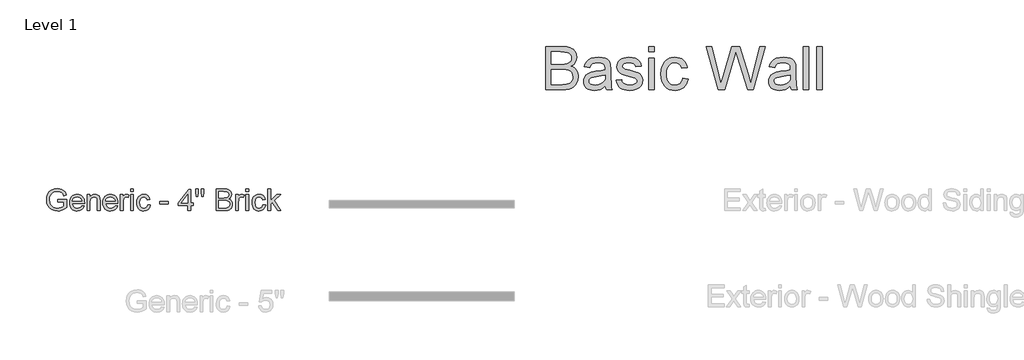
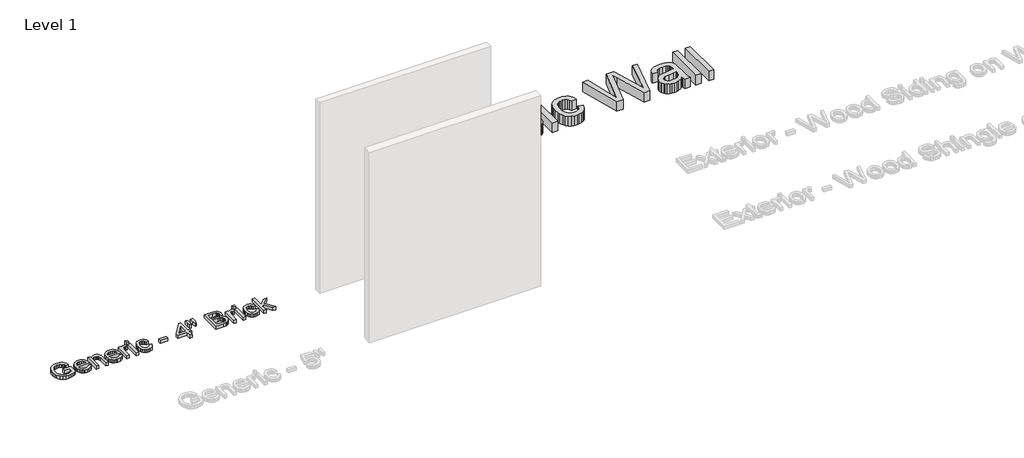
# One storey, part 29 of 42: 2 proxies.
"""IFC4 building model written with IfcOpenShell, lengths in millimetres."""

from ifc_helpers import new_model, si_unit, origin, origin_with_axes, place, context, project, spatial, polyline, outline, extrude, element, save

model = new_model("IFC4")

# Units and contexts
model_context = context("Model", 3, world=origin())
ifc_project = project(units=[si_unit("LENGTHUNIT", "METRE", prefix="MILLI")], contexts=[model_context])

# Site, building, storey
site = spatial("IfcSite", under=ifc_project)
building = spatial("IfcBuilding", under=site)
storey = spatial("IfcBuildingStorey", under=building, Name="Level 1", Elevation=0.0)

# Proxies
placement = place(None, origin())
element("IfcBuildingElementProxy", 1, Name="24\" Arial", ObjectType="24\" Arial", at=placement, inside=storey, context=model_context, shape_type="SweptSolid", body=[
    extrude(outline(polyline([(-9488.2762734, 19004.6336084), (-9488.2762734, 19613.7677966), (-9255.835664, 19613.7677966), (-9191.9070607, 19609.2877752), (-9141.9947897, 19595.8477112), (-9121.7045686, 19585.6840113), (-9103.73801, 19573.1129971), (-9088.0951139, 19558.1346685), (-9074.7758803, 19540.7490255), (-9056.5397768, 19502.6781387), (-9050.4610757, 19462.8226792), (-9055.5731332, 19426.1459899), (-9070.9093059, 19391.6628381), (-9096.5811294, 19361.4924039), (-9132.7001396, 19337.7538676), (-9109.7191173, 19327.9573064), (-9089.5543739, 19315.2236358), (-9072.2059096, 19299.5528557), (-9057.6737241, 19280.9449662), (-9046.190184, 19259.966941), (-9037.9876553, 19237.1857536), (-9033.066138, 19212.6014041), (-9031.4256323, 19186.2138926), (-9035.9056536, 19143.7373417), (-9049.3457177, 19104.3466146), (-9069.4035726, 19070.8486957), (-9093.7369665, 19046.0505692), (-9123.5356147, 19028.0933053), (-9159.9892323, 19015.1179737), (-9204.2875346, 19007.2546998), (-9257.6202368, 19004.6336084), (-9488.2762734, 19004.6336084)]), holes=[polyline([(-9412.1344999, 19366.3070326), (-9273.0865346, 19366.3070326), (-9224.4569253, 19367.9428911), (-9191.8884714, 19372.8504663), (-9163.4654314, 19384.1341715), (-9143.0357905, 19401.0318454), (-9130.7110845, 19423.2832377), (-9126.6028492, 19450.6280982), (-9130.432245, 19477.1736189), (-9141.9204325, 19500.2987083), (-9160.5469113, 19518.3489188), (-9185.7911809, 19529.6698026), (-9224.5312825, 19535.6369679), (-9283.6452571, 19537.6260231), (-9412.1344999, 19537.6260231), (-9412.1344999, 19366.3070326)]), polyline([(-9412.1344999, 19080.775382), (-9255.9843784, 19080.775382), (-9199.4729059, 19083.74967), (-9173.2434033, 19090.3488715), (-9151.6612258, 19100.3313257), (-9134.1129265, 19114.6264976), (-9119.9850583, 19134.1638521), (-9110.6718189, 19158.0696921), (-9107.5674058, 19185.4703205), (-9111.2109086, 19217.2952024), (-9122.1414171, 19244.6586523), (-9141.2326284, 19266.0549368), (-9169.3582396, 19279.9783226), (-9209.1951099, 19287.618525), (-9263.4200985, 19290.1652591), (-9412.1344999, 19290.1652591), (-9412.1344999, 19080.775382)])]), origin_with_axes(), (0.0, 0.0, 1.0), 152.4),
    extrude(outline(polyline([(-8650.7167647, 19061.7399386), (-8687.0960252, 19030.5470929), (-8724.553465, 19010.1360413), (-8763.9441921, 18998.8709254), (-8806.1233142, 18995.1158868), (-8840.0255504, 18997.3744867), (-8869.7544887, 19004.1502866), (-8895.3101291, 19015.4432865), (-8916.6924716, 19031.2534863), (-8933.5762035, 19050.5770638), (-8945.636012, 19072.4101969), (-8952.8718971, 19096.7528855), (-8955.2838588, 19123.6051296), (-8951.6403559, 19155.1697613), (-8940.7098474, 19183.8344621), (-8923.8493522, 19208.3723384), (-8902.4158891, 19227.5564961), (-8877.2273873, 19242.0561503), (-8849.1017762, 19252.5405156), (-8783.2212964, 19263.9915245), (-8705.3693072, 19276.037391), (-8651.1629079, 19290.1652591), (-8650.7167647, 19307.1187009), (-8655.9589474, 19341.0999416), (-8662.5116757, 19353.6848978), (-8671.6854953, 19363.3327446), (-8687.5421684, 19372.9620021), (-8706.8564512, 19379.8400432), (-8755.8578465, 19385.342476), (-8801.2157389, 19381.6803839), (-8832.8919064, 19370.6941075), (-8854.4926732, 19350.3760024), (-8869.6243636, 19318.7184242), (-8945.7661371, 19328.2361459), (-8932.5491447, 19369.8761783), (-8912.8258972, 19402.5933466), (-8884.7560539, 19427.6145446), (-8846.4992742, 19446.1666662), (-8799.7100056, 19457.6548537), (-8746.042696, 19461.4842495), (-8694.5689238, 19458.1009969), (-8653.7654099, 19447.951239), (-8623.0001181, 19432.6894236), (-8601.6410122, 19413.9699983), (-8587.4759655, 19390.8263196), (-8578.2928512, 19362.2917438), (-8574.5749912, 19295.667692), (-8574.5749912, 19200.9366183), (-8570.7084168, 19068.6551582), (-8564.9829123, 19035.9565792), (-8555.5395478, 19004.6336084), (-8631.6813213, 19004.6336084), (-8643.8759022, 19031.1047719), (-8650.7167647, 19061.7399386)]), holes=[polyline([(-8650.7167647, 19214.0234856), (-8701.8745188, 19201.3455829), (-8773.5548603, 19190.6753246), (-8839.0635541, 19178.3320293), (-8856.1099423, 19169.892487), (-8868.7320772, 19158.2555851), (-8876.5395832, 19144.31361), (-8879.1420853, 19128.958848), (-8873.4723487, 19106.3170804), (-8856.463139, 19087.7649588), (-8828.4862423, 19075.3844849), (-8789.9134444, 19071.2576603), (-8749.016984, 19075.8120388), (-8712.8793845, 19089.4751744), (-8683.5826474, 19109.6073865), (-8663.2087744, 19133.5689945), (-8654.1743745, 19158.2555851), (-8651.1629079, 19192.4598974), (-8650.7167647, 19214.0234856)])]), origin_with_axes(), (0.0, 0.0, 1.0), 152.4),
    extrude(outline(polyline([(-8498.4332177, 19137.8817121), (-8422.2914442, 19147.3994338), (-8417.6905924, 19130.0370274), (-8410.2827562, 19114.8309799), (-8400.0679358, 19101.7812912), (-8387.046131, 19090.8879613), (-8371.1801633, 19082.2997046), (-8352.4328541, 19076.1652355), (-8306.2942111, 19071.2576603), (-8260.713247, 19075.7562709), (-8242.997644, 19081.3795342), (-8228.6652935, 19089.2521028), (-8209.7042074, 19108.8080466), (-8204.9639358, 19119.7571444), (-8203.3838453, 19131.4869928), (-8204.9732305, 19141.7668758), (-8209.741386, 19150.8942222), (-8228.8140079, 19165.6913052), (-8257.3299944, 19175.3577412), (-8307.1864975, 19187.4036078), (-8376.6733015, 19207.4986413), (-8421.845301, 19224.6565653), (-8450.8631985, 19243.3759906), (-8471.887697, 19268.1555277), (-8484.6585462, 19297.4150862), (-8488.915496, 19329.5745755), (-8485.4950648, 19359.0757949), (-8475.2337711, 19386.3091196), (-8459.0610799, 19410.1963704), (-8437.9064563, 19429.6593676), (-8416.8819578, 19441.9097165), (-8389.4999186, 19452.1895995), (-8357.8423405, 19459.160587), (-8323.9912248, 19461.4842495), (-8274.4321506, 19457.7478002), (-8231.3421528, 19446.5384522), (-8196.6916972, 19428.9529742), (-8172.4512498, 19406.088135), (-8156.3900945, 19376.2523082), (-8146.2775152, 19337.7538676), (-8222.4192887, 19328.2361459), (-8232.0299569, 19352.1977538), (-8251.0468109, 19370.2479643), (-8279.6557439, 19381.5688481), (-8318.0426488, 19385.342476), (-8361.7646828, 19381.7361518), (-8390.9127055, 19370.9171791), (-8407.3084682, 19355.3021669), (-8412.7737225, 19337.3077244), (-8410.5058278, 19325.5964653), (-8403.702144, 19315.1492786), (-8392.0652421, 19305.8174499), (-8375.2976933, 19298.3445512), (-8309.7146423, 19282.1346815), (-8242.439965, 19262.2441303), (-8197.9557696, 19246.2945107), (-8168.435961, 19229.155176), (-8146.0544436, 19205.6954791), (-8131.9451647, 19175.8410631), (-8127.2420718, 19139.5175705), (-8132.7630939, 19101.9671842), (-8149.3261604, 19066.6475138), (-8176.2992349, 19036.3283652), (-8213.0502814, 19013.7795441), (-8257.4415302, 18999.7818011), (-8307.3352119, 18995.1158868), (-8348.3153241, 18997.3651921), (-8384.1090216, 19004.113108), (-8414.7163043, 19015.3596346), (-8440.1371723, 19031.1047719), (-8460.9014206, 19051.2741626), (-8477.5388443, 19075.7934495), (-8490.0494433, 19104.6626327), (-8498.4332177, 19137.8817121)])), origin_with_axes(), (0.0, 0.0, 1.0), 152.4),
    extrude(outline(polyline([(-8041.5825766, 19537.6260231), (-8041.5825766, 19613.7677966), (-7965.4408031, 19613.7677966), (-7965.4408031, 19537.6260231), (-8041.5825766, 19537.6260231)])), origin_with_axes(), (0.0, 0.0, 1.0), 152.4),
    extrude(outline(polyline([(-8041.5825766, 19004.6336084), (-8041.5825766, 19451.9665279), (-7965.4408031, 19451.9665279), (-7965.4408031, 19004.6336084), (-8041.5825766, 19004.6336084)])), origin_with_axes(), (0.0, 0.0, 1.0), 152.4),
    extrude(outline(polyline([(-7565.6964921, 19166.4348772), (-7489.5547186, 19156.9171555), (-7497.8362518, 19120.9886856), (-7510.7836994, 19089.1963349), (-7528.3970613, 19061.5401036), (-7550.6763375, 19038.0199916), (-7576.6827685, 19019.2494457), (-7605.4775945, 19005.841913), (-7637.0608155, 18997.7973933), (-7671.4324315, 18995.1158868), (-7714.1367013, 18998.8569834), (-7752.4260123, 19010.0802734), (-7786.3003646, 19028.7857567), (-7815.759758, 19054.9734333), (-7839.6051828, 19088.1506868), (-7856.6376291, 19127.8249007), (-7866.8570969, 19173.996075), (-7870.2635862, 19226.6642097), (-7864.4451352, 19294.4222089), (-7857.1720715, 19324.9133085), (-7846.9897823, 19353.1458081), (-7833.8285578, 19378.5527341), (-7817.6186881, 19400.5671129), (-7798.3601731, 19419.1889443), (-7776.0530129, 19434.4182285), (-7751.705677, 19446.2596127), (-7726.3266349, 19454.7177443), (-7699.9158867, 19459.7926232), (-7672.4734323, 19461.4842495), (-7638.6920266, 19459.160587), (-7608.1358644, 19452.1895995), (-7580.8049458, 19440.5712868), (-7556.6992708, 19424.3056492), (-7536.227804, 19403.7644725), (-7519.79951, 19379.3195428), (-7507.4143887, 19350.97086), (-7499.0724403, 19318.7184242), (-7575.2142138, 19309.2007025), (-7589.0260638, 19342.4197819), (-7610.5338841, 19366.2326754), (-7638.5479595, 19380.5650259), (-7671.8785747, 19385.342476), (-7697.7502332, 19382.9909296), (-7721.0844523, 19375.9362901), (-7741.8812318, 19364.1785578), (-7760.1405719, 19347.7177325), (-7775.0073647, 19326.1727336), (-7785.6265025, 19299.1624804), (-7791.9979851, 19266.686973), (-7794.1218126, 19228.7462114), (-7792.0444583, 19190.2338287), (-7785.8123955, 19157.381888), (-7775.425624, 19130.1903891), (-7760.8841439, 19108.6593322), (-7742.9872952, 19092.2961007), (-7722.5344177, 19080.6080783), (-7699.5255114, 19073.5952648), (-7673.9605763, 19071.2576603), (-7634.5326706, 19077.0947005), (-7617.4816351, 19084.3910008), (-7602.2058776, 19094.6058213), (-7589.1329523, 19107.8506977), (-7578.6904129, 19124.2371658), (-7570.8782595, 19143.7652256), (-7565.6964921, 19166.4348772)])), origin_with_axes(), (0.0, 0.0, 1.0), 152.4),
    extrude(outline(polyline([(-7066.4622466, 19004.6336084), (-7232.576233, 19613.7677966), (-7154.055029, 19613.7677966), (-7057.6880969, 19213.428628), (-7027.9452166, 19089.8469604), (-6996.1203347, 19199.1520455), (-6875.3642408, 19613.7677966), (-6762.1925813, 19613.7677966), (-6674.4510845, 19313.2159913), (-6636.8635195, 19201.6801903), (-6609.1654623, 19089.8469604), (-6580.3148684, 19209.8594824), (-6483.0556499, 19613.7677966), (-6404.534446, 19613.7677966), (-6570.7971467, 19004.6336084), (-6652.1439243, 19004.6336084), (-6798.1814665, 19474.5711169), (-6818.5553395, 19540.1541679), (-6841.4573573, 19461.1868207), (-6974.5567465, 19004.6336084), (-7066.4622466, 19004.6336084)])), origin_with_axes(), (0.0, 0.0, 1.0), 152.4),
    extrude(outline(polyline([(-6052.3787434, 19061.7399386), (-6088.7580039, 19030.5470929), (-6126.2154437, 19010.1360413), (-6165.6061708, 18998.8709254), (-6207.7852929, 18995.1158868), (-6241.6875291, 18997.3744867), (-6271.4164674, 19004.1502866), (-6296.9721078, 19015.4432865), (-6318.3544503, 19031.2534863), (-6335.2381822, 19050.5770638), (-6347.2979907, 19072.4101969), (-6354.5338758, 19096.7528855), (-6356.9458375, 19123.6051296), (-6353.3023347, 19155.1697613), (-6342.3718262, 19183.8344621), (-6325.5113309, 19208.3723384), (-6304.0778678, 19227.5564961), (-6278.8893661, 19242.0561503), (-6250.7637549, 19252.5405156), (-6184.8832751, 19263.9915245), (-6107.031286, 19276.037391), (-6052.8248866, 19290.1652591), (-6052.3787434, 19307.1187009), (-6057.6209261, 19341.0999416), (-6064.1736544, 19353.6848978), (-6073.347474, 19363.3327446), (-6089.2041471, 19372.9620021), (-6108.51843, 19379.8400432), (-6157.5198252, 19385.342476), (-6202.8777177, 19381.6803839), (-6234.5538852, 19370.6941075), (-6256.154652, 19350.3760024), (-6271.2863423, 19318.7184242), (-6347.4281158, 19328.2361459), (-6334.2111234, 19369.8761783), (-6314.4878759, 19402.5933466), (-6286.4180326, 19427.6145446), (-6248.1612529, 19446.1666662), (-6201.3719843, 19457.6548537), (-6147.7046747, 19461.4842495), (-6096.2309026, 19458.1009969), (-6055.4273887, 19447.951239), (-6024.6620969, 19432.6894236), (-6003.302991, 19413.9699983), (-5989.1379442, 19390.8263196), (-5979.95483, 19362.2917438), (-5976.2369699, 19295.667692), (-5976.2369699, 19200.9366183), (-5972.3703955, 19068.6551582), (-5966.644891, 19035.9565792), (-5957.2015265, 19004.6336084), (-6033.3433001, 19004.6336084), (-6045.537881, 19031.1047719), (-6052.3787434, 19061.7399386)]), holes=[polyline([(-6052.3787434, 19214.0234856), (-6103.5364975, 19201.3455829), (-6175.216839, 19190.6753246), (-6240.7255328, 19178.3320293), (-6257.7719211, 19169.892487), (-6270.3940559, 19158.2555851), (-6278.201562, 19144.31361), (-6280.804064, 19128.958848), (-6275.1343274, 19106.3170804), (-6258.1251178, 19087.7649588), (-6230.148221, 19075.3844849), (-6191.5754231, 19071.2576603), (-6150.6789628, 19075.8120388), (-6114.5413632, 19089.4751744), (-6085.2446261, 19109.6073865), (-6064.8707532, 19133.5689945), (-6055.8363533, 19158.2555851), (-6052.8248866, 19192.4598974), (-6052.3787434, 19214.0234856)])]), origin_with_axes(), (0.0, 0.0, 1.0), 152.4),
    extrude(outline(polyline([(-5871.5420313, 19004.6336084), (-5871.5420313, 19613.7677966), (-5795.4002578, 19613.7677966), (-5795.4002578, 19004.6336084), (-5871.5420313, 19004.6336084)])), origin_with_axes(), (0.0, 0.0, 1.0), 152.4),
    extrude(outline(polyline([(-5681.1875975, 19004.6336084), (-5681.1875975, 19613.7677966), (-5605.045824, 19613.7677966), (-5605.045824, 19004.6336084), (-5681.1875975, 19004.6336084)])), origin_with_axes(), (0.0, 0.0, 1.0), 152.4),
])
element("IfcBuildingElementProxy", 2, Name="8\" Arial", ObjectType="8\" Arial", at=placement, inside=storey, context=model_context, shape_type="SweptSolid", body=[
    extrude(outline(polyline([(-16335.8716605, 17426.1864432), (-16335.8716605, 17464.25733), (-16212.1412786, 17464.25733), (-16212.1412786, 17350.4164557), (-16242.2094716, 17329.503493), (-16273.2257189, 17314.5019278), (-16305.1156634, 17305.4675279), (-16337.8049477, 17302.4560613), (-16380.5138649, 17307.2428061), (-16419.1145467, 17321.6030404), (-16451.1810895, 17345.0348533), (-16474.2875896, 17377.0363336), (-16488.2574487, 17415.4232384), (-16492.9140684, 17458.0113251), (-16488.276038, 17500.9061353), (-16474.3619468, 17540.8080681), (-16451.7480632, 17574.2781031), (-16437.3947998, 17587.3115262), (-16421.0106553, 17597.8772196), (-16383.5718048, 17611.8749627), (-16340.853593, 17616.540877), (-16309.4934436, 17613.8361338), (-16281.2934752, 17605.7219043), (-16257.5456442, 17592.7837514), (-16239.541907, 17575.607238), (-16226.2226734, 17553.3651404), (-16216.5283534, 17525.2302346), (-16251.6249521, 17515.3407269), (-16259.4603421, 17535.4078764), (-16268.9873585, 17550.5488614), (-16281.590904, 17561.9626917), (-16298.6558816, 17570.8483772), (-16319.0018706, 17576.564587), (-16341.4484506, 17578.4699903), (-16367.7244264, 17576.4158726), (-16390.1895956, 17570.2535196), (-16408.7603065, 17560.7543872), (-16423.3529071, 17548.6899314), (-16442.9460295, 17519.3560157), (-16451.8688936, 17490.6169576), (-16454.8431816, 17459.5728263), (-16451.2647414, 17423.1656819), (-16440.5294205, 17393.2090247), (-16422.9625318, 17369.9166316), (-16398.8893881, 17353.5022795), (-16370.7173037, 17343.7707809), (-16340.853593, 17340.526948), (-16314.4846707, 17342.971441), (-16288.7663739, 17350.3049199), (-16266.4313297, 17360.4082046), (-16250.2121653, 17371.1621147), (-16250.2121653, 17426.1864432), (-16335.8716605, 17426.1864432)])), origin_with_axes(), (0.0, 0.0, 1.0), 50.8),
    extrude(outline(polyline([(-15998.4386837, 17373.8389739), (-15961.111369, 17369.0801131), (-15974.5607277, 17340.9545019), (-15996.0220747, 17319.9300034), (-16025.0120883, 17306.8245468), (-16061.0474467, 17302.4560613), (-16084.6697999, 17304.3405516), (-16105.717535, 17309.9940225), (-16124.1906521, 17319.416474), (-16140.0891511, 17332.6079061), (-16152.8739423, 17349.2011802), (-16162.005936, 17368.8291575), (-16167.4851322, 17391.4918381), (-16169.3115309, 17417.1892219), (-16167.4665429, 17443.7579792), (-16161.9315788, 17467.1758501), (-16152.7066386, 17487.4428346), (-16139.7917223, 17504.5589328), (-16123.9350492, 17518.1570058), (-16105.8848387, 17527.8699152), (-16085.6410909, 17533.6976608), (-16063.2038055, 17535.6402427), (-16041.4891793, 17533.7023081), (-16021.8519073, 17527.8885045), (-16004.2919896, 17518.1988318), (-15988.8094262, 17504.63329), (-15976.1710258, 17487.5543704), (-15967.1435969, 17467.3245645), (-15961.7271396, 17443.9438722), (-15959.9216538, 17417.4122935), (-15960.1447254, 17407.1509998), (-16131.2406442, 17407.1509998), (-16124.6507373, 17378.6536027), (-16109.3424486, 17357.7034614), (-16087.2490653, 17344.8210764), (-16060.3038747, 17340.526948), (-16040.0415375, 17342.5160031), (-16022.97656, 17348.4831685), (-16009.108942, 17358.8002301), (-15998.4386837, 17373.8389739)]), holes=[polyline([(-16131.2406442, 17445.2218866), (-15997.9925405, 17445.2218866), (-16003.1417767, 17465.3355094), (-16013.2357667, 17479.7236277), (-16035.4313911, 17493.1079239), (-16063.3525199, 17497.5693559), (-16089.0150488, 17494.0095049), (-16110.234735, 17483.329952), (-16124.9853447, 17466.6832337), (-16131.2406442, 17445.2218866)])]), origin_with_axes(), (0.0, 0.0, 1.0), 50.8),
    extrude(outline(polyline([(-15921.850767, 17307.2149221), (-15921.850767, 17530.8813818), (-15883.7798803, 17530.8813818), (-15883.7798803, 17499.6513575), (-15870.5535932, 17515.3964948), (-15854.6690362, 17526.6430214), (-15836.1262093, 17533.3909373), (-15814.9251124, 17535.6402427), (-15796.1592139, 17533.8277859), (-15778.9734059, 17528.3904156), (-15764.6410554, 17520.0066412), (-15754.4355296, 17509.3549722), (-15743.0216993, 17481.3594861), (-15741.0140549, 17444.5526718), (-15741.0140549, 17307.2149221), (-15779.0849417, 17307.2149221), (-15779.0849417, 17439.4220249), (-15783.4720165, 17473.1058369), (-15789.541423, 17483.1347643), (-15798.9754929, 17490.9143864), (-15811.0678326, 17495.9056135), (-15825.1120489, 17497.5693559), (-15847.4099145, 17493.8329066), (-15866.4174739, 17482.6235586), (-15874.0135267, 17473.4729755), (-15879.4392787, 17460.9670238), (-15883.7798803, 17425.8890144), (-15883.7798803, 17307.2149221), (-15921.850767, 17307.2149221)])), origin_with_axes(), (0.0, 0.0, 1.0), 50.8),
    extrude(outline(polyline([(-15532.0703209, 17373.8389739), (-15494.7430062, 17369.0801131), (-15508.1923649, 17340.9545019), (-15529.6537119, 17319.9300034), (-15558.6437255, 17306.8245468), (-15594.6790839, 17302.4560613), (-15618.3014371, 17304.3405516), (-15639.3491723, 17309.9940225), (-15657.8222893, 17319.416474), (-15673.7207883, 17332.6079061), (-15686.5055795, 17349.2011802), (-15695.6375732, 17368.8291575), (-15701.1167694, 17391.4918381), (-15702.9431682, 17417.1892219), (-15701.0981801, 17443.7579792), (-15695.563216, 17467.1758501), (-15686.3382758, 17487.4428346), (-15673.4233595, 17504.5589328), (-15657.5666864, 17518.1570058), (-15639.516476, 17527.8699152), (-15619.2727281, 17533.6976608), (-15596.8354428, 17535.6402427), (-15575.1208165, 17533.7023081), (-15555.4835445, 17527.8885045), (-15537.9236268, 17518.1988318), (-15522.4410635, 17504.63329), (-15509.802663, 17487.5543704), (-15500.7752341, 17467.3245645), (-15495.3587768, 17443.9438722), (-15493.553291, 17417.4122935), (-15493.7763626, 17407.1509998), (-15664.8722814, 17407.1509998), (-15658.2823745, 17378.6536027), (-15642.9740858, 17357.7034614), (-15620.8807025, 17344.8210764), (-15593.9355119, 17340.526948), (-15573.6731747, 17342.5160031), (-15556.6081972, 17348.4831685), (-15542.7405792, 17358.8002301), (-15532.0703209, 17373.8389739)]), holes=[polyline([(-15664.8722814, 17445.2218866), (-15531.6241777, 17445.2218866), (-15536.7734139, 17465.3355094), (-15546.8674039, 17479.7236277), (-15569.0630283, 17493.1079239), (-15596.9841572, 17497.5693559), (-15622.646686, 17494.0095049), (-15643.8663722, 17483.329952), (-15658.6169819, 17466.6832337), (-15664.8722814, 17445.2218866)])]), origin_with_axes(), (0.0, 0.0, 1.0), 50.8),
    extrude(outline(polyline([(-15455.4824042, 17307.2149221), (-15455.4824042, 17530.8813818), (-15422.1703783, 17530.8813818), (-15422.1703783, 17497.7924275), (-15409.8642616, 17516.9765853), (-15398.5247885, 17528.2788798), (-15387.1481368, 17533.7999019), (-15374.7304843, 17535.6402427), (-15355.7693981, 17532.7031332), (-15336.5108831, 17523.8918049), (-15349.2259644, 17489.7618498), (-15362.6102605, 17495.6174794), (-15375.9945567, 17497.5693559), (-15387.3619137, 17495.6918366), (-15397.5209663, 17490.0592786), (-15405.7281423, 17481.0992359), (-15411.2398698, 17469.2392624), (-15415.8686056, 17447.973103), (-15417.4115175, 17424.7736564), (-15417.4115175, 17307.2149221), (-15455.4824042, 17307.2149221)])), origin_with_axes(), (0.0, 0.0, 1.0), 50.8),
    extrude(outline(polyline([(-15312.7165789, 17573.7111294), (-15312.7165789, 17611.7820162), (-15274.6456921, 17611.7820162), (-15274.6456921, 17573.7111294), (-15312.7165789, 17573.7111294)])), origin_with_axes(), (0.0, 0.0, 1.0), 50.8),
    extrude(outline(polyline([(-15312.7165789, 17307.2149221), (-15312.7165789, 17530.8813818), (-15274.6456921, 17530.8813818), (-15274.6456921, 17307.2149221), (-15312.7165789, 17307.2149221)])), origin_with_axes(), (0.0, 0.0, 1.0), 50.8),
    extrude(outline(polyline([(-15074.7735366, 17388.1155565), (-15036.7026499, 17383.3566956), (-15047.3171403, 17349.4962853), (-15067.2634594, 17323.9081137), (-15094.6640878, 17307.8190744), (-15127.6415063, 17302.4560613), (-15148.9936413, 17304.3266096), (-15168.1382968, 17309.9382546), (-15185.0754729, 17319.2909962), (-15199.8051696, 17332.3848345), (-15211.727882, 17348.9734613), (-15220.2441052, 17368.8105682), (-15225.353839, 17391.8961554), (-15227.0570837, 17418.2302227), (-15224.1478582, 17452.1092223), (-15215.4201818, 17481.4710219), (-15200.7346346, 17505.1816743), (-15179.951797, 17522.1072321), (-15155.088608, 17532.25699), (-15128.1620067, 17535.6402427), (-15095.9932228, 17530.9929176), (-15070.274926, 17517.0509425), (-15051.8250456, 17494.5578893), (-15041.4615107, 17464.25733), (-15079.5323975, 17459.4984691), (-15086.4383225, 17476.1080088), (-15097.1922327, 17488.0144556), (-15111.1992703, 17495.1806308), (-15127.8645779, 17497.5693559), (-15152.4675167, 17492.8662629), (-15171.9955766, 17478.7569841), (-15184.7385418, 17454.4793581), (-15188.9861969, 17419.2712236), (-15184.8314883, 17383.5890619), (-15172.3673626, 17359.227784), (-15153.1924994, 17345.202157), (-15128.9055787, 17340.526948), (-15109.1916259, 17343.4454681), (-15093.0282294, 17352.2010285), (-15081.2704971, 17367.0167008), (-15074.7735366, 17388.1155565)])), origin_with_axes(), (0.0, 0.0, 1.0), 50.8),
    extrude(outline(polyline([(-14903.4545462, 17397.6332782), (-14903.4545462, 17435.7041649), (-14784.4830251, 17435.7041649), (-14784.4830251, 17397.6332782), (-14903.4545462, 17397.6332782)])), origin_with_axes(), (0.0, 0.0, 1.0), 50.8),
    extrude(outline(polyline([(-14508.4690961, 17307.2149221), (-14508.4690961, 17378.5978348), (-14646.4760606, 17378.5978348), (-14646.4760606, 17416.6687215), (-14498.9513744, 17607.0231553), (-14470.3982093, 17607.0231553), (-14470.3982093, 17416.6687215), (-14432.3273226, 17416.6687215), (-14432.3273226, 17378.5978348), (-14470.3982093, 17378.5978348), (-14470.3982093, 17307.2149221), (-14508.4690961, 17307.2149221)]), holes=[polyline([(-14508.4690961, 17416.6687215), (-14508.4690961, 17534.301813), (-14599.6310242, 17416.6687215), (-14508.4690961, 17416.6687215)])]), origin_with_axes(), (0.0, 0.0, 1.0), 50.8),
    extrude(outline(polyline([(-14389.7206466, 17502.3282167), (-14399.0152967, 17561.1447625), (-14399.0152967, 17611.7820162), (-14360.9444099, 17611.7820162), (-14360.9444099, 17561.1447625), (-14369.2724164, 17502.3282167), (-14389.7206466, 17502.3282167)])), origin_with_axes(), (0.0, 0.0, 1.0), 50.8),
    extrude(outline(polyline([(-14313.8019447, 17502.3282167), (-14322.8735232, 17561.1447625), (-14322.8735232, 17611.7820162), (-14284.8026364, 17611.7820162), (-14284.8026364, 17561.1447625), (-14293.7255005, 17502.3282167), (-14313.8019447, 17502.3282167)])), origin_with_axes(), (0.0, 0.0, 1.0), 50.8),
    extrude(outline(polyline([(-14113.483646, 17307.2149221), (-14113.483646, 17611.7820162), (-13997.2633413, 17611.7820162), (-13965.2990396, 17609.5420055), (-13940.3429042, 17602.8219735), (-13921.2145143, 17591.4546164), (-13906.7334494, 17575.2726306), (-13897.6153977, 17556.2371872), (-13894.5760471, 17536.3094575), (-13897.1320759, 17517.9711128), (-13904.8001622, 17500.7295369), (-13917.636074, 17485.6443198), (-13935.6955791, 17473.7750517), (-13914.1226963, 17462.5099358), (-13898.1823714, 17445.370601), (-13888.3393369, 17423.4909947), (-13885.0583254, 17398.0050642), (-13887.2983361, 17376.7667887), (-13894.0183681, 17357.0714252), (-13904.0472956, 17340.3224657), (-13916.2139925, 17327.9234025), (-13931.1133166, 17318.9447705), (-13949.3401254, 17312.4571048), (-13998.1556277, 17307.2149221), (-14113.483646, 17307.2149221)]), holes=[polyline([(-14075.4127592, 17488.0516342), (-14005.8887766, 17488.0516342), (-13965.289745, 17491.323351), (-13951.078225, 17496.9652036), (-13940.8634046, 17505.4140406), (-13934.7010516, 17516.5397367), (-13932.6469339, 17530.212167), (-13934.5616318, 17543.4849273), (-13940.3057256, 17555.047472), (-13949.6189649, 17564.0725773), (-13962.2410998, 17569.7330192), (-14011.1681378, 17573.7111294), (-14075.4127592, 17573.7111294), (-14075.4127592, 17488.0516342)]), polyline([(-14075.4127592, 17345.2858089), (-13997.3376985, 17345.2858089), (-13969.0819622, 17346.7729529), (-13945.1761222, 17355.0637808), (-13929.3380385, 17371.9800439), (-13924.6814188, 17383.9329639), (-13923.1292122, 17397.6332782), (-13924.9509636, 17413.5457191), (-13930.4162179, 17427.227444), (-13939.9618235, 17437.9255863), (-13954.0246291, 17444.8872792), (-13973.9430642, 17448.7073804), (-14001.0555585, 17449.9807474), (-14075.4127592, 17449.9807474), (-14075.4127592, 17345.2858089)])]), origin_with_axes(), (0.0, 0.0, 1.0), 50.8),
    extrude(outline(polyline([(-13837.469717, 17307.2149221), (-13837.469717, 17530.8813818), (-13804.1576911, 17530.8813818), (-13804.1576911, 17497.7924275), (-13791.8515744, 17516.9765853), (-13780.5121012, 17528.2788798), (-13769.1354495, 17533.7999019), (-13756.717797, 17535.6402427), (-13737.7567108, 17532.7031332), (-13718.4981959, 17523.8918049), (-13731.2132772, 17489.7618498), (-13744.5975733, 17495.6174794), (-13757.9818694, 17497.5693559), (-13769.3492265, 17495.6918366), (-13779.508279, 17490.0592786), (-13787.7154551, 17481.0992359), (-13793.2271826, 17469.2392624), (-13797.8559183, 17447.973103), (-13799.3988302, 17424.7736564), (-13799.3988302, 17307.2149221), (-13837.469717, 17307.2149221)])), origin_with_axes(), (0.0, 0.0, 1.0), 50.8),
    extrude(outline(polyline([(-13694.7038916, 17573.7111294), (-13694.7038916, 17611.7820162), (-13656.6330049, 17611.7820162), (-13656.6330049, 17573.7111294), (-13694.7038916, 17573.7111294)])), origin_with_axes(), (0.0, 0.0, 1.0), 50.8),
    extrude(outline(polyline([(-13694.7038916, 17307.2149221), (-13694.7038916, 17530.8813818), (-13656.6330049, 17530.8813818), (-13656.6330049, 17307.2149221), (-13694.7038916, 17307.2149221)])), origin_with_axes(), (0.0, 0.0, 1.0), 50.8),
    extrude(outline(polyline([(-13456.7608494, 17388.1155565), (-13418.6899626, 17383.3566956), (-13429.304453, 17349.4962853), (-13449.2507721, 17323.9081137), (-13476.6514006, 17307.8190744), (-13509.6288191, 17302.4560613), (-13530.980954, 17304.3266096), (-13550.1256095, 17309.9382546), (-13567.0627857, 17319.2909962), (-13581.7924824, 17332.3848345), (-13593.7151948, 17348.9734613), (-13602.2314179, 17368.8105682), (-13607.3411518, 17391.8961554), (-13609.0443964, 17418.2302227), (-13606.135171, 17452.1092223), (-13597.4074945, 17481.4710219), (-13582.7219474, 17505.1816743), (-13561.9391098, 17522.1072321), (-13537.0759208, 17532.25699), (-13510.1493195, 17535.6402427), (-13477.9805356, 17530.9929176), (-13452.2622388, 17517.0509425), (-13433.8123583, 17494.5578893), (-13423.4488235, 17464.25733), (-13461.5197102, 17459.4984691), (-13468.4256353, 17476.1080088), (-13479.1795454, 17488.0144556), (-13493.1865831, 17495.1806308), (-13509.8518907, 17497.5693559), (-13534.4548295, 17492.8662629), (-13553.9828893, 17478.7569841), (-13566.7258546, 17454.4793581), (-13570.9735097, 17419.2712236), (-13566.8188011, 17383.5890619), (-13554.3546753, 17359.227784), (-13535.1798122, 17345.202157), (-13510.8928915, 17340.526948), (-13491.1789387, 17343.4454681), (-13475.0155422, 17352.2010285), (-13463.2578098, 17367.0167008), (-13456.7608494, 17388.1155565)])), origin_with_axes(), (0.0, 0.0, 1.0), 50.8),
    extrude(outline(polyline([(-13385.3779367, 17307.2149221), (-13385.3779367, 17611.7820162), (-13347.30705, 17611.7820162), (-13347.30705, 17448.1218174), (-13261.9449836, 17530.8813818), (-13209.3000855, 17530.8813818), (-13295.7031527, 17447.0808166), (-13204.5412246, 17307.2149221), (-13249.0068306, 17307.2149221), (-13322.9922453, 17420.6096532), (-13347.30705, 17397.0384205), (-13347.30705, 17307.2149221), (-13385.3779367, 17307.2149221)])), origin_with_axes(), (0.0, 0.0, 1.0), 50.8),
])

save(model, "model.ifc")

# Revit data of these elements
# Element 1 (IfcBuildingElementProxy, "24\" Arial")
#   Phase Created = New Construction
# Element 2 (IfcBuildingElementProxy, "8\" Arial")
#   Phase Created = New Construction
